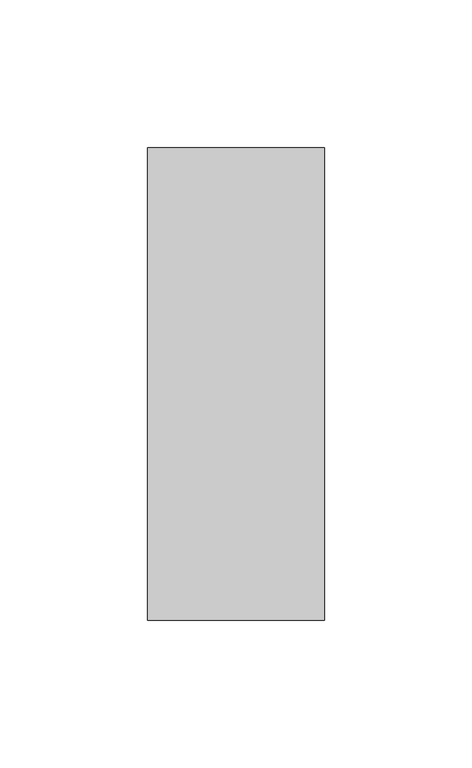
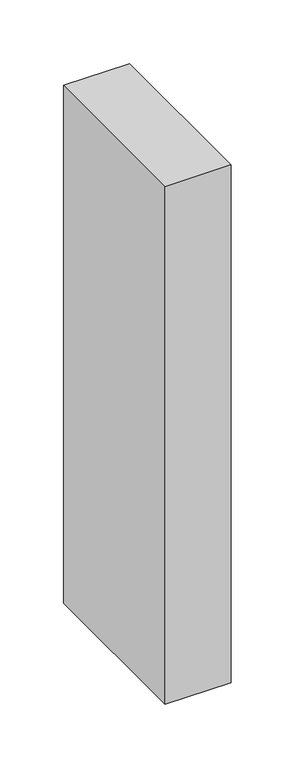
"""IFC4 building model written with IfcOpenShell, lengths in millimetres: column geometry, Madeira de lei-Coluna : Pontalete 6X16cm."""

import ifcopenshell
import ifcopenshell.guid

model = None  # the IFC model being written
_history = None  # IfcOwnerHistory: only IFC2X3 demands one
_inside = {}  # id of a spatial element -> (the spatial element, [elements in it])
_under = {}  # id of a project, library or spatial element -> (it, [spatial elements below it])
_declared = {}  # id of a project -> (the project, [libraries it declares])
_typed = {}  # id of a type object -> (the type object, [elements of that type])
_made_of = {}  # id of a material, layer set ... -> (it, [elements and type objects made of it])


def new_model(schema):
    """Start an empty IFC model of exactly this schema.

    Asked for "IFC4X3", IfcOpenShell would pick the latest addendum, in which some entities
    have other attributes; the version numbers below select the first issue.
    IFC2X3 requires an IfcOwnerHistory on every rooted entity: one is made here for all.
    """
    global model, _history
    if schema == "IFC4X3":
        model = ifcopenshell.file(schema_version=(4, 3, 0, 0))
    else:
        model = ifcopenshell.file(schema=schema)
    _inside.clear()
    _under.clear()
    _declared.clear()
    _typed.clear()
    _made_of.clear()
    _history = None
    if model.schema == "IFC2X3":
        org = make("IfcOrganization", Name="unknown")
        user = make(
            "IfcPersonAndOrganization",
            ThePerson=make("IfcPerson", FamilyName="unknown"),
            TheOrganization=org,
        )
        app = make(
            "IfcApplication",
            ApplicationDeveloper=org,
            Version="unknown",
            ApplicationFullName="unknown",
            ApplicationIdentifier="unknown",
        )
        _history = make(
            "IfcOwnerHistory",
            OwningUser=user,
            OwningApplication=app,
            ChangeAction="ADDED",
            CreationDate=0,
        )
    return model


def make(cls, **values):
    """One entity of the class cls with the attributes given. An attribute that is None is left unset."""
    return model.create_entity(
        cls, **{name: value for name, value in values.items() if value is not None}
    )


def rooted(cls, **values):
    """An entity with a GlobalId (a new one), such as an element, a storey or a relation."""
    return make(cls, GlobalId=ifcopenshell.guid.new(), OwnerHistory=_history, **values)


def si_unit(unit_type, name, prefix=None):
    """IfcSIUnit, for example si_unit("LENGTHUNIT", "METRE", prefix="MILLI")."""
    return make("IfcSIUnit", UnitType=unit_type, Prefix=prefix, Name=name)


def assignment(units):
    """IfcUnitAssignment: the units of a project."""
    return None if units is None else make("IfcUnitAssignment", Units=units)


def point(xyz):
    """IfcCartesianPoint."""
    return None if xyz is None else make("IfcCartesianPoint", Coordinates=xyz)


def direction(xyz):
    """IfcDirection."""
    return None if xyz is None else make("IfcDirection", DirectionRatios=xyz)


def frame(location, z_axis=None, x_axis=None):
    """IfcAxis2Placement3D, a coordinate frame: its origin and axes. An axis left out is left unset."""
    return make(
        "IfcAxis2Placement3D",
        Location=point(location),
        Axis=direction(z_axis),
        RefDirection=direction(x_axis),
    )


def origin():
    """The frame at (0, 0, 0) with its axes left unset."""
    return frame((0.0, 0.0, 0.0))


def place(relative_to, where):
    """IfcLocalPlacement: puts the frame where relative to a parent placement (None: the world)."""
    return make(
        "IfcLocalPlacement", PlacementRelTo=relative_to, RelativePlacement=where
    )


def context(
    kind, dimensions, precision=None, world=None, true_north=None, identifier=None
):
    """IfcGeometricRepresentationContext, for example the 3D "Model" context."""
    return make(
        "IfcGeometricRepresentationContext",
        ContextIdentifier=identifier,
        ContextType=kind,
        CoordinateSpaceDimension=dimensions,
        Precision=precision,
        WorldCoordinateSystem=world,
        TrueNorth=true_north,
    )


def project(units=None, contexts=None):
    """IfcProject with its units and contexts."""
    return rooted(
        "IfcProject",
        Name="project",
        RepresentationContexts=contexts,
        UnitsInContext=assignment(units),
    )


def spatial(cls, under=None, at=None, **own):
    """A site, building, storey or space (cls), placed at a placement, below another one or the project."""
    s = rooted(cls, ObjectPlacement=at, **own)
    if under is not None:
        _under.setdefault(under.id(), (under, []))[1].append(s)
    return s


def polyline(points):
    """IfcPolyline through the points."""
    return make("IfcPolyline", Points=[point(p) for p in points])


def outline(outer, holes=None, kind="AREA"):
    """IfcArbitraryClosedProfileDef: a profile drawn as a closed curve; with holes, ...WithVoids."""
    if holes is None:
        return make("IfcArbitraryClosedProfileDef", ProfileType=kind, OuterCurve=outer)
    return make(
        "IfcArbitraryProfileDefWithVoids",
        ProfileType=kind,
        OuterCurve=outer,
        InnerCurves=holes,
    )


def extrude(swept, where, along, depth):
    """IfcExtrudedAreaSolid: the profile swept, set in the frame where, extruded along a direction by depth."""
    return make(
        "IfcExtrudedAreaSolid",
        SweptArea=swept,
        Position=where,
        ExtrudedDirection=direction(along),
        Depth=depth,
    )


def shape(context_of_items, identifier, shape_type, items):
    """IfcShapeRepresentation: the items that make up one representation, for example the "Body"."""
    return make(
        "IfcShapeRepresentation",
        ContextOfItems=context_of_items,
        RepresentationIdentifier=identifier,
        RepresentationType=shape_type,
        Items=items,
    )


def source(mapping_origin, context_of_items, identifier, shape_type, items):
    """IfcRepresentationMap: a shape defined once, which mapped items show again and again."""
    return make(
        "IfcRepresentationMap",
        MappingOrigin=mapping_origin,
        MappedRepresentation=shape(context_of_items, identifier, shape_type, items),
    )


def transform(
    local_origin,
    x_axis=None,
    y_axis=None,
    z_axis=None,
    scale=None,
    scale2=None,
    scale3=None,
    uniform=True,
):
    """IfcCartesianTransformationOperator3D, or its non-uniform kind. x_axis, y_axis, z_axis: its Axis1, 2, 3."""
    if uniform:
        return make(
            "IfcCartesianTransformationOperator3D",
            Axis1=direction(x_axis),
            Axis2=direction(y_axis),
            LocalOrigin=point(local_origin),
            Scale=scale,
            Axis3=direction(z_axis),
        )
    return make(
        "IfcCartesianTransformationOperator3DnonUniform",
        Axis1=direction(x_axis),
        Axis2=direction(y_axis),
        LocalOrigin=point(local_origin),
        Scale=scale,
        Axis3=direction(z_axis),
        Scale2=scale2,
        Scale3=scale3,
    )


def mapped(mapping_source, mapping_target):
    """IfcMappedItem: shows the shape of a source again, moved by a transform."""
    return make(
        "IfcMappedItem", MappingSource=mapping_source, MappingTarget=mapping_target
    )


def made_of(thing, what):
    """Note that an element or type object is made of a material, layer set ...; save() writes the relation."""
    if what is not None:
        _made_of.setdefault(what.id(), (what, []))[1].append(thing)
    return thing


def element(
    cls,
    number,
    at=None,
    inside=None,
    cuts=None,
    type_object=None,
    material=None,
    context=None,
    identifier="Body",
    shape_type=None,
    held_by="IfcProductDefinitionShape",
    body=None,
    shapes=None,
    **own,
):
    """One element of the class cls, such as IfcWall. Its Tag is "e" and its number.

    at: its placement. inside: the storey or other place that contains it. cuts: it is an
    opening in that element (IfcRelVoidsElement). A single representation is given by context,
    identifier, shape_type and body (its items); several are given by shapes. held_by: the class
    of the entity that holds the representations. save() writes the other relations.
    """
    e = rooted(cls, Tag="e%d" % number, ObjectPlacement=at, **own)
    if body is not None:
        shapes = [shape(context, identifier, shape_type, body)]
    if shapes is not None:
        e.Representation = make(held_by, Representations=shapes)
    if inside is not None:
        _inside.setdefault(inside.id(), (inside, []))[1].append(e)
    if cuts is not None:
        rooted(
            "IfcRelVoidsElement", RelatingBuildingElement=cuts, RelatedOpeningElement=e
        )
    if type_object is not None:
        _typed.setdefault(type_object.id(), (type_object, []))[1].append(e)
    return made_of(e, material)


def aggregate(whole, parts):
    """IfcRelAggregates: a whole, such as a stair, and the parts it consists of."""
    return rooted("IfcRelAggregates", RelatingObject=whole, RelatedObjects=parts)


def save(model, path):
    """Write the relations noted so far, then the file.

    IfcRelAggregates (storeys below a building ...), IfcRelContainedInSpatialStructure (elements
    in a storey), IfcRelDefinesByType, IfcRelAssociatesMaterial and IfcRelDeclares: one each for
    every whole, place, type object, material and project.
    """
    for whole, parts in _under.values():
        aggregate(whole, parts)
    for where, things in _inside.values():
        rooted(
            "IfcRelContainedInSpatialStructure",
            RelatedElements=things,
            RelatingStructure=where,
        )
    for kind, things in _typed.values():
        rooted("IfcRelDefinesByType", RelatedObjects=things, RelatingType=kind)
    for what, things in _made_of.values():
        rooted("IfcRelAssociatesMaterial", RelatedObjects=things, RelatingMaterial=what)
    for by, libraries in _declared.values():
        rooted("IfcRelDeclares", RelatingContext=by, RelatedDefinitions=libraries)
    model.write(path)


def column_924cc83b(model_context):
    return source(origin(), model_context, "Body", "SweptSolid", [
        extrude(outline(polyline([(30.0, 80.0), (30.0, -80.0), (-30.0, -80.0), (-30.0, 80.0), (30.0, 80.0)])), frame((0.0, 0.0, 4460.0), z_axis=(0.0, 0.0, 1.0), x_axis=(1.0, 0.0, 0.0)), (0.0, 0.0, 1.0), 497.0),
    ])


if __name__ == "__main__":
    model = new_model("IFC4")
    model_context = context("Model", 3, world=origin())
    ifc_project = project(units=[si_unit("LENGTHUNIT", "METRE", prefix="MILLI")], contexts=[model_context])
    site = spatial("IfcSite", under=ifc_project)
    building = spatial("IfcBuilding", under=site)
    placement = place(None, origin())
    column_shape = column_924cc83b(model_context)
    element("IfcColumn", 1, ObjectType="Madeira de lei-Coluna : Pontalete 6X16cm", at=placement, inside=building, context=model_context, shape_type="MappedRepresentation", body=[
        mapped(column_shape, transform((0.0, 0.0, 0.0), x_axis=(1.0, 0.0, 0.0), y_axis=(0.0, 1.0, 0.0), z_axis=(0.0, 0.0, 1.0))),
    ])
    save(model, "model.ifc")

# Revit data of these elements
# Type "Madeira de lei-Coluna : Pontalete 6X16cm"
#   A = 0.01952 m²
#   b = 0.06 m
#   d = 0.16 m
#   Structural Material [instance default] = none
#   Assembly Code = ""
# Element 1 (IfcColumn, "Madeira de lei-Coluna : Pontalete 6X16cm")
#   Structural Material = .MADEIRAMENTO
#   Materials on its faces: ".MADEIRAMENTO"
# Materials
#   ".MADEIRAMENTO": class ".CC_MADEIRAS", colour RGB 212 179 113, transparency 0, Cost = 0
